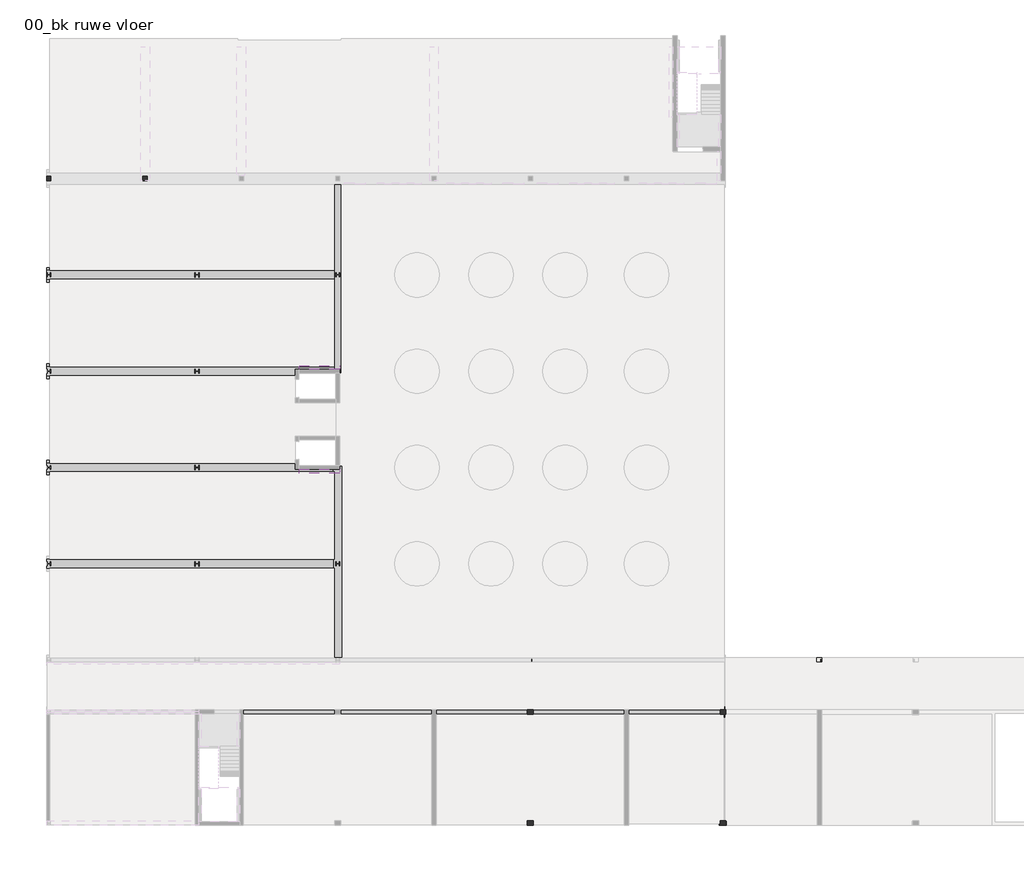
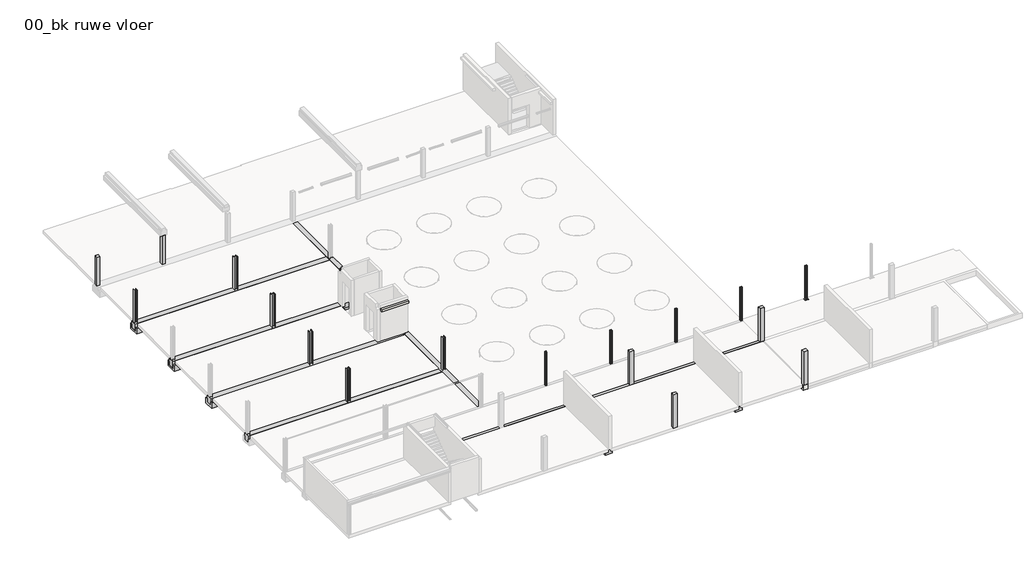
# One storey, part 5 of 6: 17 columns, 12 beams, 2 footings, 2 walls.
"""IFC4 building model written with IfcOpenShell, lengths in millimetres."""

import ifcopenshell
import ifcopenshell.guid

model = None  # the IFC model being written
_history = None  # IfcOwnerHistory: only IFC2X3 demands one
_inside = {}  # id of a spatial element -> (the spatial element, [elements in it])
_under = {}  # id of a project, library or spatial element -> (it, [spatial elements below it])
_declared = {}  # id of a project -> (the project, [libraries it declares])
_typed = {}  # id of a type object -> (the type object, [elements of that type])
_made_of = {}  # id of a material, layer set ... -> (it, [elements and type objects made of it])


def new_model(schema):
    """Start an empty IFC model of exactly this schema.

    Asked for "IFC4X3", IfcOpenShell would pick the latest addendum, in which some entities
    have other attributes; the version numbers below select the first issue.
    IFC2X3 requires an IfcOwnerHistory on every rooted entity: one is made here for all.
    """
    global model, _history
    if schema == "IFC4X3":
        model = ifcopenshell.file(schema_version=(4, 3, 0, 0))
    else:
        model = ifcopenshell.file(schema=schema)
    _inside.clear()
    _under.clear()
    _declared.clear()
    _typed.clear()
    _made_of.clear()
    _history = None
    if model.schema == "IFC2X3":
        org = make("IfcOrganization", Name="unknown")
        user = make(
            "IfcPersonAndOrganization",
            ThePerson=make("IfcPerson", FamilyName="unknown"),
            TheOrganization=org,
        )
        app = make(
            "IfcApplication",
            ApplicationDeveloper=org,
            Version="unknown",
            ApplicationFullName="unknown",
            ApplicationIdentifier="unknown",
        )
        _history = make(
            "IfcOwnerHistory",
            OwningUser=user,
            OwningApplication=app,
            ChangeAction="ADDED",
            CreationDate=0,
        )
    return model


def make(cls, **values):
    """One entity of the class cls with the attributes given. An attribute that is None is left unset."""
    return model.create_entity(
        cls, **{name: value for name, value in values.items() if value is not None}
    )


def rooted(cls, **values):
    """An entity with a GlobalId (a new one), such as an element, a storey or a relation."""
    return make(cls, GlobalId=ifcopenshell.guid.new(), OwnerHistory=_history, **values)


def si_unit(unit_type, name, prefix=None):
    """IfcSIUnit, for example si_unit("LENGTHUNIT", "METRE", prefix="MILLI")."""
    return make("IfcSIUnit", UnitType=unit_type, Prefix=prefix, Name=name)


def assignment(units):
    """IfcUnitAssignment: the units of a project."""
    return None if units is None else make("IfcUnitAssignment", Units=units)


def point(xyz):
    """IfcCartesianPoint."""
    return None if xyz is None else make("IfcCartesianPoint", Coordinates=xyz)


def direction(xyz):
    """IfcDirection."""
    return None if xyz is None else make("IfcDirection", DirectionRatios=xyz)


def frame(location, z_axis=None, x_axis=None):
    """IfcAxis2Placement3D, a coordinate frame: its origin and axes. An axis left out is left unset."""
    return make(
        "IfcAxis2Placement3D",
        Location=point(location),
        Axis=direction(z_axis),
        RefDirection=direction(x_axis),
    )


def frame_2d(location, x_axis=None):
    """IfcAxis2Placement2D, a coordinate frame in the plane: its origin and x axis."""
    return make(
        "IfcAxis2Placement2D", Location=point(location), RefDirection=direction(x_axis)
    )


def origin():
    """The frame at (0, 0, 0) with its axes left unset."""
    return frame((0.0, 0.0, 0.0))


def place(relative_to, where):
    """IfcLocalPlacement: puts the frame where relative to a parent placement (None: the world)."""
    return make(
        "IfcLocalPlacement", PlacementRelTo=relative_to, RelativePlacement=where
    )


def context(
    kind, dimensions, precision=None, world=None, true_north=None, identifier=None
):
    """IfcGeometricRepresentationContext, for example the 3D "Model" context."""
    return make(
        "IfcGeometricRepresentationContext",
        ContextIdentifier=identifier,
        ContextType=kind,
        CoordinateSpaceDimension=dimensions,
        Precision=precision,
        WorldCoordinateSystem=world,
        TrueNorth=true_north,
    )


def project(units=None, contexts=None):
    """IfcProject with its units and contexts."""
    return rooted(
        "IfcProject",
        Name="project",
        RepresentationContexts=contexts,
        UnitsInContext=assignment(units),
    )


def spatial(cls, under=None, at=None, **own):
    """A site, building, storey or space (cls), placed at a placement, below another one or the project."""
    s = rooted(cls, ObjectPlacement=at, **own)
    if under is not None:
        _under.setdefault(under.id(), (under, []))[1].append(s)
    return s


def polyline(points):
    """IfcPolyline through the points."""
    return make("IfcPolyline", Points=[point(p) for p in points])


def circle_curve(where, radius):
    """IfcCircle in the frame where."""
    return make("IfcCircle", Position=where, Radius=radius)


def trimmed(basis, trim1, trim2, sense, master):
    """IfcTrimmedCurve: the piece of a basis curve between two trims."""
    return make(
        "IfcTrimmedCurve",
        BasisCurve=basis,
        Trim1=trim1,
        Trim2=trim2,
        SenseAgreement=sense,
        MasterRepresentation=master,
    )


def segment(curve, same_sense, transition):
    """IfcCompositeCurveSegment."""
    return make(
        "IfcCompositeCurveSegment",
        Transition=transition,
        SameSense=same_sense,
        ParentCurve=curve,
    )


def composite_curve(segments, self_intersect=None):
    """IfcCompositeCurve: segments joined end to end."""
    return make("IfcCompositeCurve", Segments=segments, SelfIntersect=self_intersect)


def outline(outer, holes=None, kind="AREA"):
    """IfcArbitraryClosedProfileDef: a profile drawn as a closed curve; with holes, ...WithVoids."""
    if holes is None:
        return make("IfcArbitraryClosedProfileDef", ProfileType=kind, OuterCurve=outer)
    return make(
        "IfcArbitraryProfileDefWithVoids",
        ProfileType=kind,
        OuterCurve=outer,
        InnerCurves=holes,
    )


def extrude(swept, where, along, depth):
    """IfcExtrudedAreaSolid: the profile swept, set in the frame where, extruded along a direction by depth."""
    return make(
        "IfcExtrudedAreaSolid",
        SweptArea=swept,
        Position=where,
        ExtrudedDirection=direction(along),
        Depth=depth,
    )


def faces_of(points, faces, orient=None, outer=None):
    """IfcFace entities. A face is a list of loops; a loop is a list of indices into points, from 0.

    orient and outer hold one flag for each loop. By default every Orientation is true, the
    first loop of a face is its IfcFaceOuterBound and the others are IfcFaceBound.
    """
    made = []
    for i, loops in enumerate(faces):
        bounds = []
        for j, loop in enumerate(loops):
            is_outer = j == 0 if outer is None else outer[i][j]
            bounds.append(
                make(
                    "IfcFaceOuterBound" if is_outer else "IfcFaceBound",
                    Bound=make("IfcPolyLoop", Polygon=[points[k] for k in loop]),
                    Orientation=True if orient is None else orient[i][j],
                )
            )
        made.append(make("IfcFace", Bounds=bounds))
    return made


def faceted_brep(points, faces, orient=None, outer=None, voids=None):
    """IfcFacetedBrep: a solid bounded by flat faces; with voids (closed shells), ...WithVoids."""
    shared = [point(p) for p in points]
    hull = make("IfcClosedShell", CfsFaces=faces_of(shared, faces, orient, outer))
    if voids is None:
        return make("IfcFacetedBrep", Outer=hull)
    return make(
        "IfcFacetedBrepWithVoids",
        Outer=hull,
        Voids=[
            make(cls, CfsFaces=faces_of(shared, fs, o, b)) for cls, fs, o, b in voids
        ],
    )


def shape(context_of_items, identifier, shape_type, items):
    """IfcShapeRepresentation: the items that make up one representation, for example the "Body"."""
    return make(
        "IfcShapeRepresentation",
        ContextOfItems=context_of_items,
        RepresentationIdentifier=identifier,
        RepresentationType=shape_type,
        Items=items,
    )


def source(mapping_origin, context_of_items, identifier, shape_type, items):
    """IfcRepresentationMap: a shape defined once, which mapped items show again and again."""
    return make(
        "IfcRepresentationMap",
        MappingOrigin=mapping_origin,
        MappedRepresentation=shape(context_of_items, identifier, shape_type, items),
    )


def transform(
    local_origin,
    x_axis=None,
    y_axis=None,
    z_axis=None,
    scale=None,
    scale2=None,
    scale3=None,
    uniform=True,
):
    """IfcCartesianTransformationOperator3D, or its non-uniform kind. x_axis, y_axis, z_axis: its Axis1, 2, 3."""
    if uniform:
        return make(
            "IfcCartesianTransformationOperator3D",
            Axis1=direction(x_axis),
            Axis2=direction(y_axis),
            LocalOrigin=point(local_origin),
            Scale=scale,
            Axis3=direction(z_axis),
        )
    return make(
        "IfcCartesianTransformationOperator3DnonUniform",
        Axis1=direction(x_axis),
        Axis2=direction(y_axis),
        LocalOrigin=point(local_origin),
        Scale=scale,
        Axis3=direction(z_axis),
        Scale2=scale2,
        Scale3=scale3,
    )


def mapped(mapping_source, mapping_target):
    """IfcMappedItem: shows the shape of a source again, moved by a transform."""
    return make(
        "IfcMappedItem", MappingSource=mapping_source, MappingTarget=mapping_target
    )


def made_of(thing, what):
    """Note that an element or type object is made of a material, layer set ...; save() writes the relation."""
    if what is not None:
        _made_of.setdefault(what.id(), (what, []))[1].append(thing)
    return thing


def element(
    cls,
    number,
    at=None,
    inside=None,
    cuts=None,
    type_object=None,
    material=None,
    context=None,
    identifier="Body",
    shape_type=None,
    held_by="IfcProductDefinitionShape",
    body=None,
    shapes=None,
    **own,
):
    """One element of the class cls, such as IfcWall. Its Tag is "e" and its number.

    at: its placement. inside: the storey or other place that contains it. cuts: it is an
    opening in that element (IfcRelVoidsElement). A single representation is given by context,
    identifier, shape_type and body (its items); several are given by shapes. held_by: the class
    of the entity that holds the representations. save() writes the other relations.
    """
    e = rooted(cls, Tag="e%d" % number, ObjectPlacement=at, **own)
    if body is not None:
        shapes = [shape(context, identifier, shape_type, body)]
    if shapes is not None:
        e.Representation = make(held_by, Representations=shapes)
    if inside is not None:
        _inside.setdefault(inside.id(), (inside, []))[1].append(e)
    if cuts is not None:
        rooted(
            "IfcRelVoidsElement", RelatingBuildingElement=cuts, RelatedOpeningElement=e
        )
    if type_object is not None:
        _typed.setdefault(type_object.id(), (type_object, []))[1].append(e)
    return made_of(e, material)


def aggregate(whole, parts):
    """IfcRelAggregates: a whole, such as a stair, and the parts it consists of."""
    return rooted("IfcRelAggregates", RelatingObject=whole, RelatedObjects=parts)


def save(model, path):
    """Write the relations noted so far, then the file.

    IfcRelAggregates (storeys below a building ...), IfcRelContainedInSpatialStructure (elements
    in a storey), IfcRelDefinesByType, IfcRelAssociatesMaterial and IfcRelDeclares: one each for
    every whole, place, type object, material and project.
    """
    for whole, parts in _under.values():
        aggregate(whole, parts)
    for where, things in _inside.values():
        rooted(
            "IfcRelContainedInSpatialStructure",
            RelatedElements=things,
            RelatingStructure=where,
        )
    for kind, things in _typed.values():
        rooted("IfcRelDefinesByType", RelatedObjects=things, RelatingType=kind)
    for what, things in _made_of.values():
        rooted("IfcRelAssociatesMaterial", RelatedObjects=things, RelatingMaterial=what)
    for by, libraries in _declared.values():
        rooted("IfcRelDeclares", RelatingContext=by, RelatedDefinitions=libraries)
    model.write(path)


def column_d8346d76(model_context):
    return source(origin(), model_context, "Body", "SweptSolid", [
        extrude(outline(composite_curve([segment(trimmed(circle_curve(frame_2d((60.0, 60.0)), 20.0), [point((60.0, 80.0))], [point((80.0, 60.0))], False, "CARTESIAN"), True, "CONTINUOUS"), segment(polyline([(80.0, 60.0), (80.0, -60.0)]), True, "CONTINUOUS"), segment(trimmed(circle_curve(frame_2d((60.0, -60.0)), 20.0), [point((80.0, -60.0))], [point((60.0, -80.0))], False, "CARTESIAN"), True, "CONTINUOUS"), segment(polyline([(60.0, -80.0), (-60.0, -80.0)]), True, "CONTINUOUS"), segment(trimmed(circle_curve(frame_2d((-60.0, -60.0)), 20.0), [point((-60.0, -80.0))], [point((-80.0, -60.0))], False, "CARTESIAN"), True, "CONTINUOUS"), segment(polyline([(-80.0, -60.0), (-80.0, 60.0)]), True, "CONTINUOUS"), segment(trimmed(circle_curve(frame_2d((-60.0, 60.0)), 20.0), [point((-80.0, 60.0))], [point((-60.0, 80.0))], False, "CARTESIAN"), True, "CONTINUOUS"), segment(polyline([(-60.0, 80.0), (60.0, 80.0)]), True, "CONTINUOUS")], self_intersect=False), holes=[composite_curve([segment(polyline([(60.0, 72.0), (-60.0, 72.0)]), True, "CONTINUOUS"), segment(trimmed(circle_curve(frame_2d((-60.0, 60.0)), 12.0), [point((-60.0, 72.0))], [point((-72.0, 60.0))], True, "CARTESIAN"), True, "CONTINUOUS"), segment(polyline([(-72.0, 60.0), (-72.0, -60.0)]), True, "CONTINUOUS"), segment(trimmed(circle_curve(frame_2d((-60.0, -60.0)), 12.0), [point((-72.0, -60.0))], [point((-60.0, -72.0))], True, "CARTESIAN"), True, "CONTINUOUS"), segment(polyline([(-60.0, -72.0), (60.0, -72.0)]), True, "CONTINUOUS"), segment(trimmed(circle_curve(frame_2d((60.0, -60.0)), 12.0), [point((60.0, -72.0))], [point((72.0, -60.0))], True, "CARTESIAN"), True, "CONTINUOUS"), segment(polyline([(72.0, -60.0), (72.0, 60.0)]), True, "CONTINUOUS"), segment(trimmed(circle_curve(frame_2d((60.0, 60.0)), 12.0), [point((72.0, 60.0))], [point((60.0, 72.0))], True, "CARTESIAN"), True, "CONTINUOUS")], self_intersect=False)]), frame((0.0, 0.0, -40.0), z_axis=(0.0, 0.0, 1.0), x_axis=(1.0, 0.0, 0.0)), (0.0, 0.0, 1.0), 3510.0),
    ])


model = new_model("IFC4")

# Units and contexts
model_context = context("Model", 3, world=origin())
ifc_project = project(units=[si_unit("LENGTHUNIT", "METRE", prefix="MILLI")], contexts=[model_context])

# Site, building, storey
site = spatial("IfcSite", under=ifc_project)
building = spatial("IfcBuilding", under=site)
storey = spatial("IfcBuildingStorey", under=building, Name="00_bk ruwe vloer", Elevation=-70.0)

# Beams
placement = place(None, origin())
element("IfcBeam", 1, ObjectType="NLRS_28_SF_LIB_balk dubbele sponning beton prefab-CWV-MMBC-SRP_gen_rsf : balk beton prefab_gen__bxh 700x700 met inkassing bxh 200x320", at=placement, inside=storey, context=model_context, shape_type="Brep", body=[
    faceted_brep([(52150.0, 7650.0, -70.0), (52150.0, 7350.0, -70.0), (52150.0, 7350.0, -390.0), (52150.0, 7150.0, -390.0), (52150.0, 7150.0, -770.0), (52150.0, 7850.0, -770.0), (52150.0, 7850.0, -390.0), (52150.0, 7650.0, -390.0), (52090.0, 7650.0, -70.0), (51800.0, 7650.0, -70.0), (39200.0, 7650.0, -70.0), (38800.0, 7650.0, -70.0), (26200.0, 7650.0, -70.0), (25800.0, 7650.0, -70.0), (19625.0, 7650.0, -70.0), (19375.0, 7650.0, -70.0), (19375.0, 7400.0, -70.0), (19375.0, 7350.0, -70.0), (25800.0, 7350.0, -70.0), (26200.0, 7350.0, -70.0), (32350.0, 7350.0, -70.0), (32650.0, 7350.0, -70.0), (38800.0, 7350.0, -70.0), (39200.0, 7350.0, -70.0), (45350.0, 7350.0, -70.0), (45650.0, 7350.0, -70.0), (51800.0, 7350.0, -70.0), (52050.0, 7350.0, -70.0), (19375.0, 7350.0, -390.0), (19625.0, 7350.0, -390.0), (32350.0, 7350.0, -390.0), (32650.0, 7350.0, -390.0), (45350.0, 7350.0, -390.0), (45650.0, 7350.0, -390.0), (52050.0, 7350.0, -390.0), (19625.0, 7175.0, -390.0), (19625.0, 7150.0, -390.0), (32150.0, 7150.0, -390.0), (32175.0, 7150.0, -390.0), (32350.0, 7150.0, -390.0), (32650.0, 7150.0, -390.0), (32825.0, 7150.0, -390.0), (32850.0, 7150.0, -390.0), (45150.0, 7150.0, -390.0), (45175.0, 7150.0, -390.0), (45350.0, 7150.0, -390.0), (45650.0, 7150.0, -390.0), (45825.0, 7150.0, -390.0), (45850.0, 7150.0, -390.0), (51850.0, 7150.0, -390.0), (51875.0, 7150.0, -390.0), (52050.0, 7150.0, -390.0), (19625.0, 7150.0, -770.0), (32150.0, 7150.0, -770.0), (32850.0, 7150.0, -770.0), (45150.0, 7150.0, -770.0), (45850.0, 7150.0, -770.0), (51850.0, 7150.0, -770.0), (19625.0, 7650.0, -770.0), (19375.0, 7650.0, -770.0), (19375.0, 7850.0, -770.0), (51850.0, 7850.0, -770.0), (19375.0, 7850.0, -390.0), (51850.0, 7850.0, -390.0), (51875.0, 7850.0, -390.0), (52090.0, 7850.0, -390.0), (19375.0, 7825.0, -390.0), (19375.0, 7650.0, -390.0), (19625.0, 7650.0, -390.0), (52090.0, 7650.0, -390.0), (19625.0, 7650.0, -390.0)], [[[0, 1, 2, 3, 4, 5, 6, 7]], [[1, 0, 8, 9, 10, 11, 12, 13, 14, 15, 16, 17, 18, 19, 20, 21, 22, 23, 24, 25, 26, 27]], [[2, 1, 27, 26, 25, 24, 23, 22, 21, 20, 19, 18, 17, 28, 29, 30, 31, 32, 33, 34]], [[3, 2, 34, 33, 32, 31, 30, 29, 35, 36, 37, 38, 39, 40, 41, 42, 43, 44, 45, 46, 47, 48, 49, 50, 51]], [[4, 3, 51, 50, 49, 48, 47, 46, 45, 44, 43, 42, 41, 40, 39, 38, 37, 36, 52, 53, 54, 55, 56, 57]], [[5, 4, 57, 56, 55, 54, 53, 52, 58, 59, 60, 61]], [[6, 5, 61, 60, 62, 63, 64, 65]], [[7, 6, 65, 64, 63, 62, 66, 67, 68, 69]], [[0, 7, 69, 68, 67, 15, 14, 13, 12, 11, 10, 9, 8]], [[17, 16, 15, 67, 28]], [[29, 70, 58, 52, 36, 35]], [[67, 70, 29, 28]], [[70, 67, 59, 58]], [[62, 60, 59, 67, 66]]]),
])
element("IfcBeam", 2, ObjectType="NLRS_28_SF_LIB_balk dubbele sponning beton ihwg-CWV-MMBC-SRP_gen_rsf : balk beton ihwg_gen__bxh 1000x900 met inkassing bxh 200x320", at=placement, inside=storey, context=model_context, shape_type="Brep", body=[
    faceted_brep([(6350.0, 17200.0, -70.0), (6350.0, 17800.0, -70.0), (6350.0, 17800.0, -390.0), (6350.0, 17800.0, -770.0), (6350.0, 17200.0, -770.0), (6350.0, 17200.0, -390.0), (6550.0, 17200.0, -70.0), (25700.0, 17200.0, -70.0), (25700.0, 17800.0, -70.0), (6550.0, 17800.0, -70.0), (25500.0, 17200.0, -770.0), (25500.0, 17200.0, -390.0), (25550.0, 17200.0, -390.0), (25700.0, 17200.0, -390.0), (25700.0, 17800.0, -390.0), (25550.0, 17800.0, -390.0), (25500.0, 17800.0, -390.0), (25500.0, 17800.0, -770.0)], [[[0, 1, 2, 3, 4, 5]], [[1, 0, 6, 7, 8, 9]], [[0, 5, 4, 10, 11, 12, 13, 7, 6]], [[3, 2, 1, 9, 8, 14, 15, 16, 17]], [[4, 3, 17, 10]], [[16, 11, 10, 17]], [[14, 13, 12, 11, 16, 15]], [[13, 14, 8, 7]]]),
])
element("IfcBeam", 3, ObjectType="NLRS_28_SF_LIB_balk dubbele sponning beton ihwg-CWV-MMBC-SRP_gen_rsf : balk beton ihwg_gen__bxh 1000x900 met inkassing bxh 200x320", at=placement, inside=storey, context=model_context, shape_type="Brep", body=[
    faceted_brep([(6350.0, 23700.0, -70.0), (6350.0, 24300.0, -70.0), (6350.0, 24300.0, -390.0), (6350.0, 24300.0, -770.0), (6350.0, 23700.0, -770.0), (6350.0, 23700.0, -390.0), (6550.0, 23700.0, -70.0), (25700.0, 23700.0, -70.0), (25700.0, 23875.0, -70.0), (23375.0, 23875.0, -70.0), (23125.0, 23875.0, -70.0), (23125.0, 24300.0, -70.0), (6550.0, 24300.0, -70.0), (25500.0, 23700.0, -770.0), (25500.0, 23700.0, -390.0), (25550.0, 23700.0, -390.0), (25700.0, 23700.0, -390.0), (23125.0, 24300.0, -390.0), (23125.0, 24300.0, -770.0), (23125.0, 23875.0, -770.0), (23375.0, 23875.0, -770.0), (25500.0, 23875.0, -770.0), (25500.0, 23875.0, -390.0), (25700.0, 23875.0, -390.0)], [[[0, 1, 2, 3, 4, 5]], [[1, 0, 6, 7, 8, 9, 10, 11, 12]], [[0, 5, 4, 13, 14, 15, 16, 7, 6]], [[3, 2, 1, 12, 11, 17, 18]], [[4, 3, 18, 19, 20, 21, 13]], [[17, 11, 10, 19, 18]], [[22, 14, 13, 21]], [[14, 22, 23, 16, 15]], [[16, 23, 8, 7]], [[19, 10, 9, 8, 23, 22, 21, 20]]]),
])
element("IfcBeam", 4, ObjectType="NLRS_28_SF_LIB_balk dubbele sponning beton ihwg-CWV-MMBC-SRP_gen_rsf : balk beton ihwg_gen__bxh 1000x900 met inkassing bxh 200x320", at=placement, inside=storey, context=model_context, shape_type="Brep", body=[
    faceted_brep([(25750.0, 30800.0, -390.0), (25750.0, 30800.0, -70.0), (25750.0, 30625.0, -70.0), (25750.0, 30625.0, -390.0), (6350.0, 30200.0, -70.0), (6350.0, 30800.0, -70.0), (6350.0, 30800.0, -390.0), (6350.0, 30800.0, -770.0), (6350.0, 30200.0, -770.0), (6350.0, 30200.0, -390.0), (6550.0, 30200.0, -70.0), (23125.0, 30200.0, -70.0), (23375.0, 30200.0, -70.0), (23375.0, 30375.0, -70.0), (23375.0, 30625.0, -70.0), (6550.0, 30800.0, -70.0), (23375.0, 30200.0, -770.0), (23375.0, 30200.0, -390.0), (25550.0, 30800.0, -390.0), (25550.0, 30800.0, -770.0), (25550.0, 30625.0, -770.0), (23375.0, 30625.0, -770.0), (25550.0, 30625.0, -390.0)], [[[0, 1, 2, 3]], [[4, 5, 6, 7, 8, 9]], [[5, 4, 10, 11, 12, 13, 14, 2, 1, 15]], [[4, 9, 8, 16, 17, 12, 11, 10]], [[1, 0, 18, 19, 7, 6, 5, 15]], [[7, 19, 20, 21, 16, 8]], [[14, 21, 20, 22, 3, 2]], [[21, 14, 13, 12, 17, 16]], [[18, 22, 20, 19]], [[22, 18, 0, 3]]]),
])
element("IfcBeam", 5, ObjectType="NLRS_28_SF_LIB_balk dubbele sponning beton ihwg-CWV-MMBC-SRP_gen_rsf : balk beton ihwg_gen__bxh 1000x900 met inkassing bxh 200x320", at=placement, inside=storey, context=model_context, shape_type="Brep", body=[
    faceted_brep([(6350.0, 36700.0, -70.0), (6350.0, 37300.0, -70.0), (6350.0, 37300.0, -390.0), (6350.0, 37300.0, -770.0), (6350.0, 36700.0, -770.0), (6350.0, 36700.0, -390.0), (6550.0, 36700.0, -70.0), (25750.0, 36700.0, -70.0), (25750.0, 37300.0, -70.0), (6550.0, 37300.0, -70.0), (25550.0, 36700.0, -770.0), (25550.0, 36700.0, -390.0), (25750.0, 36700.0, -390.0), (25550.0, 37300.0, -770.0), (25750.0, 37300.0, -390.0), (25550.0, 37300.0, -390.0)], [[[0, 1, 2, 3, 4, 5]], [[1, 0, 6, 7, 8, 9]], [[4, 10, 11, 12, 7, 6, 0, 5]], [[13, 3, 2, 1, 9, 8, 14, 15]], [[3, 13, 10, 4]], [[15, 11, 10, 13]], [[11, 15, 14, 12]], [[12, 14, 8, 7]]]),
])
element("IfcBeam", 6, ObjectType="NLRS_28_SF_LIB_balkbodem beton prefab-CWV-MMBC-SRP_gen_rsf : balkbodem beton prefab_gen__bxhxdk 1000x580x200", at=placement, inside=storey, context=model_context, shape_type="Brep", body=[
    faceted_brep([(25550.0, 36500.0, -390.0), (25550.0, 36500.0, -970.0), (25550.0, 37500.0, -970.0), (25550.0, 37500.0, -390.0), (25550.0, 37300.0, -390.0), (25550.0, 37300.0, -770.0), (25550.0, 36700.0, -770.0), (25550.0, 36700.0, -390.0), (6350.0, 36500.0, -390.0), (6350.0, 36700.0, -390.0), (6350.0, 36700.0, -770.0), (6350.0, 37300.0, -770.0), (6350.0, 37300.0, -390.0), (6350.0, 37500.0, -390.0), (6350.0, 37500.0, -970.0), (6350.0, 36500.0, -970.0), (6650.0, 36500.0, -390.0), (6550.0, 36500.0, -390.0), (6650.0, 36500.0, -970.0), (6650.0, 37500.0, -970.0), (6550.0, 37500.0, -390.0), (6650.0, 37500.0, -390.0), (6550.0, 37300.0, -390.0), (6550.0, 36700.0, -390.0)], [[[0, 1, 2, 3, 4, 5, 6, 7]], [[8, 9, 10, 11, 12, 13, 14, 15]], [[1, 0, 16, 17, 8, 15, 18]], [[2, 1, 18, 15, 14, 19]], [[3, 2, 19, 14, 13, 20, 21]], [[4, 3, 21, 20, 13, 12, 22]], [[5, 4, 22, 12, 11]], [[6, 5, 11, 10]], [[7, 6, 10, 9, 23]], [[0, 7, 23, 9, 8, 17, 16]]]),
])
element("IfcBeam", 7, ObjectType="NLRS_28_SF_LIB_balkbodem beton prefab-CWV-MMBC-SRP_gen_rsf : balkbodem beton prefab_gen__bxhxdk 1000x580x200", at=placement, inside=storey, context=model_context, shape_type="Brep", body=[
    faceted_brep([(25550.0, 31000.0, -970.0), (25550.0, 31000.0, -390.0), (25550.0, 30800.0, -390.0), (25550.0, 30800.0, -770.0), (25550.0, 30625.0, -770.0), (25550.0, 30625.0, -970.0), (6350.0, 30000.0, -390.0), (6350.0, 30200.0, -390.0), (6350.0, 30200.0, -770.0), (6350.0, 30800.0, -770.0), (6350.0, 30800.0, -390.0), (6350.0, 31000.0, -390.0), (6350.0, 31000.0, -970.0), (6350.0, 30000.0, -970.0), (6650.0, 30000.0, -970.0), (23125.0, 30000.0, -970.0), (23375.0, 30000.0, -970.0), (23375.0, 30000.0, -390.0), (23125.0, 30000.0, -390.0), (6650.0, 30000.0, -390.0), (6550.0, 30000.0, -390.0), (6650.0, 31000.0, -970.0), (23375.0, 30625.0, -970.0), (6550.0, 31000.0, -390.0), (6650.0, 31000.0, -390.0), (6550.0, 30800.0, -390.0), (23375.0, 30200.0, -770.0), (23375.0, 30625.0, -770.0), (6550.0, 30200.0, -390.0), (23125.0, 30200.0, -390.0), (23375.0, 30200.0, -390.0)], [[[0, 1, 2, 3, 4, 5]], [[6, 7, 8, 9, 10, 11, 12, 13]], [[6, 13, 14, 15, 16, 17, 18, 19, 20]], [[13, 12, 21, 0, 5, 22, 16, 15, 14]], [[1, 0, 21, 12, 11, 23, 24]], [[2, 1, 24, 23, 11, 10, 25]], [[3, 2, 25, 10, 9]], [[9, 8, 26, 27, 4, 3]], [[8, 7, 28, 29, 30, 26]], [[7, 6, 20, 19, 18, 17, 30, 29, 28]], [[27, 22, 5, 4]], [[17, 16, 22, 27, 26, 30]]]),
])
element("IfcBeam", 8, ObjectType="NLRS_28_SF_LIB_balkbodem beton prefab-CWV-MMBC-SRP_gen_rsf : balkbodem beton prefab_gen__bxhxdk 1000x580x200", at=placement, inside=storey, context=model_context, shape_type="Brep", body=[
    faceted_brep([(25550.0, 23500.0, -390.0), (25550.0, 23500.0, -970.0), (25550.0, 23875.0, -970.0), (25550.0, 23875.0, -770.0), (25550.0, 23700.0, -770.0), (25550.0, 23700.0, -390.0), (6350.0, 23500.0, -390.0), (6350.0, 23700.0, -390.0), (6350.0, 23700.0, -770.0), (6350.0, 24300.0, -770.0), (6350.0, 24300.0, -390.0), (6350.0, 24500.0, -390.0), (6350.0, 24500.0, -970.0), (6350.0, 23500.0, -970.0), (25500.0, 23500.0, -390.0), (6650.0, 23500.0, -390.0), (6550.0, 23500.0, -390.0), (6650.0, 23500.0, -970.0), (25500.0, 23500.0, -970.0), (6650.0, 24500.0, -970.0), (23125.0, 24500.0, -970.0), (23375.0, 24500.0, -970.0), (23375.0, 23875.0, -970.0), (6550.0, 24500.0, -390.0), (6650.0, 24500.0, -390.0), (23125.0, 24500.0, -390.0), (23375.0, 24500.0, -390.0), (6550.0, 24300.0, -390.0), (23125.0, 24300.0, -390.0), (23375.0, 24300.0, -390.0), (23125.0, 24300.0, -770.0), (23375.0, 24300.0, -770.0), (25500.0, 23700.0, -770.0), (25500.0, 23875.0, -770.0), (23375.0, 23875.0, -770.0), (6550.0, 23700.0, -390.0), (25500.0, 23700.0, -390.0)], [[[0, 1, 2, 3, 4, 5]], [[6, 7, 8, 9, 10, 11, 12, 13]], [[1, 0, 14, 15, 16, 6, 13, 17, 18]], [[13, 12, 19, 20, 21, 22, 2, 1, 18, 17]], [[12, 11, 23, 24, 25, 26, 21, 20, 19]], [[11, 10, 27, 28, 29, 26, 25, 24, 23]], [[10, 9, 30, 31, 29, 28, 27]], [[9, 8, 32, 4, 3, 33, 34, 31, 30]], [[5, 4, 32, 8, 7, 35, 36]], [[0, 5, 36, 35, 7, 6, 16, 15, 14]], [[22, 34, 33, 3, 2]], [[21, 26, 29, 31, 34, 22]]]),
])
element("IfcBeam", 9, ObjectType="NLRS_28_SF_LIB_balk dubbele sponning beton ihwg-CWV-MMBC-SRP_gen_rsf : balk beton ihwg_gen__bxh 900x900 met inkassing bxh 200x320", at=placement, inside=storey, context=model_context, shape_type="Brep", body=[
    faceted_brep([(25750.0, 43100.0, -70.0), (26250.0, 43100.0, -70.0), (26250.0, 43100.0, -390.0), (25750.0, 43100.0, -390.0), (25750.0, 30375.0, -70.0), (25750.0, 30375.0, -390.0), (25550.0, 30375.0, -390.0), (25550.0, 30375.0, -970.0), (25875.0, 30375.0, -970.0), (25875.0, 30375.0, -390.0), (26125.0, 30375.0, -390.0), (26125.0, 30375.0, -970.0), (26450.0, 30375.0, -970.0), (26450.0, 30375.0, -390.0), (26425.0, 30375.0, -390.0), (26250.0, 30375.0, -390.0), (26250.0, 30375.0, -70.0), (25750.0, 37300.0, -70.0), (25750.0, 36700.0, -70.0), (25750.0, 30800.0, -70.0), (25750.0, 30625.0, -70.0), (26250.0, 42900.0, -390.0), (26450.0, 42900.0, -390.0), (26425.0, 42900.0, -390.0), (26450.0, 42900.0, -970.0), (26125.0, 30625.0, -970.0), (25875.0, 30625.0, -970.0), (25550.0, 30625.0, -970.0), (25550.0, 36500.0, -970.0), (25550.0, 37500.0, -970.0), (25550.0, 42900.0, -970.0), (25550.0, 30625.0, -390.0), (25550.0, 30800.0, -390.0), (25550.0, 36500.0, -390.0), (25550.0, 36700.0, -390.0), (25550.0, 37300.0, -390.0), (25550.0, 37500.0, -390.0), (25550.0, 42900.0, -390.0), (25750.0, 30625.0, -390.0), (25750.0, 30800.0, -390.0), (25750.0, 36700.0, -390.0), (25750.0, 37300.0, -390.0), (25750.0, 42900.0, -390.0), (26125.0, 30625.0, -390.0), (25875.0, 30625.0, -390.0)], [[[0, 1, 2, 3]], [[4, 5, 6, 7, 8, 9, 10, 11, 12, 13, 14, 15, 16]], [[1, 0, 17, 18, 19, 20, 4, 16]], [[2, 1, 16, 15, 21]], [[21, 15, 14, 13, 22, 23]], [[13, 12, 24, 22]], [[12, 11, 25, 26, 8, 7, 27, 28, 29, 30, 24]], [[7, 6, 31, 32, 33, 34, 35, 36, 37, 30, 29, 28, 27]], [[6, 5, 38, 39, 40, 41, 42, 37, 36, 35, 34, 33, 32, 31]], [[0, 3, 42, 41, 40, 39, 38, 5, 4, 20, 19, 18, 17]], [[3, 2, 21, 42]], [[22, 24, 30, 37, 42, 21, 23]], [[10, 43, 25, 11]], [[26, 44, 9, 8]], [[43, 44, 26, 25]], [[44, 43, 10, 9]]]),
])
element("IfcBeam", 10, ObjectType="NLRS_28_SF_LIB_balk dubbele sponning beton ihwg-CWV-MMBC-SRP_gen_rsf : balk beton ihwg_gen__bxh 1000x900 met inkassing bxh 200x320", at=placement, inside=storey, context=model_context, shape_type="Brep", body=[
    faceted_brep([(26300.0, 24125.0, -70.0), (26300.0, 24125.0, -390.0), (26425.0, 24125.0, -390.0), (26500.0, 24125.0, -390.0), (26500.0, 24125.0, -970.0), (26125.0, 24125.0, -970.0), (26125.0, 24125.0, -390.0), (25875.0, 24125.0, -390.0), (25875.0, 24125.0, -70.0), (26300.0, 11150.0, -390.0), (26300.0, 11150.0, -70.0), (25750.0, 11150.0, -70.0), (25750.0, 11150.0, -390.0), (25875.0, 23875.0, -70.0), (25700.0, 23875.0, -70.0), (25700.0, 23700.0, -70.0), (25750.0, 23700.0, -70.0), (25750.0, 17800.0, -70.0), (25700.0, 17800.0, -70.0), (25700.0, 17200.0, -70.0), (25750.0, 17200.0, -70.0), (26300.0, 11350.0, -390.0), (26425.0, 11350.0, -390.0), (26500.0, 11350.0, -390.0), (26500.0, 11350.0, -970.0), (26125.0, 23875.0, -970.0), (25500.0, 11350.0, -970.0), (25500.0, 17000.0, -970.0), (25550.0, 17000.0, -970.0), (25550.0, 18000.0, -970.0), (25500.0, 18000.0, -970.0), (25500.0, 23500.0, -970.0), (25550.0, 23500.0, -970.0), (25550.0, 23875.0, -970.0), (25500.0, 23875.0, -390.0), (25500.0, 23875.0, -770.0), (25500.0, 23700.0, -770.0), (25500.0, 23700.0, -390.0), (25750.0, 11350.0, -390.0), (25750.0, 17200.0, -390.0), (25700.0, 17200.0, -390.0), (25700.0, 17800.0, -390.0), (25750.0, 17800.0, -390.0), (25750.0, 23700.0, -390.0), (25700.0, 23700.0, -390.0), (25700.0, 23875.0, -390.0), (25550.0, 23700.0, -390.0), (25550.0, 23500.0, -390.0), (25500.0, 23500.0, -390.0), (25500.0, 18000.0, -390.0), (25550.0, 18000.0, -390.0), (25550.0, 17800.0, -390.0), (25500.0, 17800.0, -390.0), (25500.0, 17200.0, -390.0), (25550.0, 17200.0, -390.0), (25550.0, 17000.0, -390.0), (25500.0, 17000.0, -390.0), (25500.0, 11350.0, -390.0), (25550.0, 23700.0, -770.0), (25550.0, 23875.0, -770.0), (25550.0, 17200.0, -770.0), (25550.0, 17800.0, -770.0), (25500.0, 17800.0, -770.0), (25500.0, 17200.0, -770.0), (25875.0, 23875.0, -390.0), (26125.0, 23875.0, -390.0)], [[[0, 1, 2, 3, 4, 5, 6, 7, 8]], [[9, 10, 11, 12]], [[10, 0, 8, 13, 14, 15, 16, 17, 18, 19, 20, 11]], [[1, 0, 10, 9, 21]], [[1, 21, 22, 23, 3, 2]], [[4, 3, 23, 24]], [[25, 5, 4, 24, 26, 27, 28, 29, 30, 31, 32, 33]], [[34, 35, 36, 37]], [[38, 39, 40, 41, 42, 43, 44, 45, 34, 37, 46, 47, 48, 49, 50, 51, 52, 53, 54, 55, 56, 57]], [[44, 15, 14, 45]], [[24, 23, 22, 21, 38, 57, 26]], [[12, 38, 21, 9]], [[32, 47, 46, 58, 59, 33]], [[47, 32, 31, 48]], [[58, 46, 37, 36]], [[28, 55, 54, 60, 61, 51, 50, 29]], [[55, 28, 27, 56]], [[29, 50, 49, 30]], [[51, 61, 62, 52]], [[60, 54, 53, 63]], [[20, 39, 38, 12, 11]], [[39, 20, 19, 40]], [[43, 42, 17, 16]], [[17, 42, 41, 18]], [[43, 16, 15, 44]], [[45, 14, 13, 64, 65, 25, 33, 59, 35, 34]], [[25, 65, 6, 5]], [[65, 64, 7, 6]], [[58, 36, 35, 59]], [[61, 60, 63, 62]], [[48, 31, 30, 49]], [[53, 52, 62, 63]], [[26, 57, 56, 27]], [[40, 19, 18, 41]], [[13, 8, 7, 64]]]),
])
element("IfcBeam", 11, ObjectType="NLRS_28_SF_LIB_balk dubbele sponning beton prefab-CWV-MMBC-SRP_gen_rsf : balk beton prefab_gen__bxh 700x700 met inkassing bxh 200x320", at=placement, inside=storey, context=model_context, shape_type="Brep", body=[
    faceted_brep([(32650.0, 7350.0, -70.0), (32350.0, 7350.0, -70.0), (32350.0, 150.0, -70.0), (32650.0, 150.0, -70.0), (32350.0, 7350.0, -390.0), (32350.0, 7150.0, -390.0), (32350.0, 150.0, -390.0), (32850.0, 7150.0, -390.0), (32825.0, 7150.0, -390.0), (32650.0, 7150.0, -390.0), (32650.0, 150.0, -390.0), (32850.0, 150.0, -390.0), (32150.0, 7150.0, -390.0), (32150.0, 7150.0, -770.0), (32150.0, 150.0, -770.0), (32150.0, 150.0, -390.0), (32850.0, 7150.0, -770.0), (32850.0, 150.0, -770.0), (32650.0, 7350.0, -390.0), (32175.0, 7150.0, -390.0)], [[[0, 1, 2, 3]], [[1, 4, 5, 6, 2]], [[7, 8, 9, 10, 11]], [[12, 13, 14, 15]], [[13, 16, 17, 14]], [[16, 7, 11, 17]], [[18, 0, 3, 10, 9]], [[1, 0, 18, 4]], [[5, 4, 18, 9]], [[13, 12, 19, 5, 9, 8, 7, 16]], [[19, 12, 15, 6, 5]], [[3, 2, 6, 15, 14, 17, 11, 10]]]),
])
element("IfcBeam", 12, ObjectType="NLRS_28_SF_LIB_balk dubbele sponning beton prefab-CWV-MMBC-SRP_gen_rsf : balk beton prefab_gen__bxh 700x700 met inkassing bxh 200x320", at=placement, inside=storey, context=model_context, shape_type="Brep", body=[
    faceted_brep([(45650.0, 7350.0, -70.0), (45350.0, 7350.0, -70.0), (45350.0, 150.0, -70.0), (45650.0, 150.0, -70.0), (45350.0, 7350.0, -390.0), (45350.0, 7150.0, -390.0), (45350.0, 150.0, -390.0), (45850.0, 7150.0, -390.0), (45825.0, 7150.0, -390.0), (45650.0, 7150.0, -390.0), (45650.0, 150.0, -390.0), (45850.0, 150.0, -390.0), (45150.0, 7150.0, -390.0), (45150.0, 7150.0, -770.0), (45150.0, 150.0, -770.0), (45150.0, 150.0, -390.0), (45850.0, 7150.0, -770.0), (45850.0, 150.0, -770.0), (45650.0, 7350.0, -390.0), (45175.0, 7150.0, -390.0)], [[[0, 1, 2, 3]], [[1, 4, 5, 6, 2]], [[7, 8, 9, 10, 11]], [[12, 13, 14, 15]], [[13, 16, 17, 14]], [[16, 7, 11, 17]], [[18, 0, 3, 10, 9]], [[1, 0, 18, 4]], [[5, 4, 18, 9]], [[13, 12, 19, 5, 9, 8, 7, 16]], [[19, 12, 15, 6, 5]], [[3, 2, 6, 15, 14, 17, 11, 10]]]),
])

# Columns
element("IfcColumn", 13, ObjectType="NLRS_28_SCO_TLB_stalen kolom HEA-BCPG-MMBS-SRP_gen_rsf : stalen kolom_gen__HEA 260", at=placement, inside=storey, context=model_context, shape_type="SweptSolid", body=[
    extrude(outline(composite_curve([segment(polyline([(6375.0, 37130.0), (6387.5, 37130.0), (6387.5, 37027.75)]), True, "CONTINUOUS"), segment(trimmed(circle_curve(frame_2d((6411.5, 37027.75)), 24.0), [point((6387.5, 37027.75))], [point((6411.5, 37003.75))], True, "CARTESIAN"), True, "CONTINUOUS"), segment(polyline([(6411.5, 37003.75), (6588.5, 37003.75)]), True, "CONTINUOUS"), segment(trimmed(circle_curve(frame_2d((6588.5, 37027.75)), 24.0), [point((6588.5, 37003.75))], [point((6612.5, 37027.75))], True, "CARTESIAN"), True, "CONTINUOUS"), segment(polyline([(6612.5, 37027.75), (6612.5, 37130.0), (6625.0, 37130.0), (6625.0, 36870.0), (6612.5, 36870.0), (6612.5, 36972.25)]), True, "CONTINUOUS"), segment(trimmed(circle_curve(frame_2d((6588.5, 36972.25)), 24.0), [point((6612.5, 36972.25))], [point((6588.5, 36996.25))], True, "CARTESIAN"), True, "CONTINUOUS"), segment(polyline([(6588.5, 36996.25), (6411.5, 36996.25)]), True, "CONTINUOUS"), segment(trimmed(circle_curve(frame_2d((6411.5, 36972.25)), 24.0), [point((6411.5, 36996.25))], [point((6387.5, 36972.25))], True, "CARTESIAN"), True, "CONTINUOUS"), segment(polyline([(6387.5, 36972.25), (6387.5, 36870.0), (6375.0, 36870.0), (6375.0, 37130.0)]), True, "CONTINUOUS")], self_intersect=False)), frame((0.0, 0.0, -40.0), z_axis=(0.0, 0.0, 1.0), x_axis=(1.0, 0.0, 0.0)), (0.0, 0.0, 1.0), 3420.0),
])
element("IfcColumn", 14, ObjectType="NLRS_28_SCO_TLB_vierkante kolom beton prefab-BCPG-MMBPC-SRP_gen_rsf : kolom vierkant beton prefab_gen__bxh 300x300", at=placement, inside=storey, context=model_context, shape_type="SweptSolid", body=[
    extrude(outline(polyline([(6350.0, 43650.0), (6650.0, 43650.0), (6650.0, 43350.0), (6350.0, 43350.0), (6350.0, 43650.0)])), frame((0.0, 0.0, -40.0), z_axis=(0.0, 0.0, 1.0), x_axis=(1.0, 0.0, 0.0)), (0.0, 0.0, 1.0), 3020.0),
])
element("IfcColumn", 15, ObjectType="NLRS_28_SCO_TLB_vierkante kolom beton prefab-BCPG-MMBPC-SRP_gen_rsf : kolom vierkant beton prefab_gen__bxh 300x300", at=placement, inside=storey, context=model_context, shape_type="SweptSolid", body=[
    extrude(outline(polyline([(13150.0, 43650.0), (13150.0, 43350.0), (12850.0, 43350.0), (12850.0, 43650.0), (13150.0, 43650.0)])), frame((0.0, 0.0, -40.0), z_axis=(0.0, 0.0, 1.0), x_axis=(1.0, 0.0, 0.0)), (0.0, 0.0, 1.0), 3020.0),
])
element("IfcColumn", 16, ObjectType="NLRS_28_SCO_TLB_stalen kolom HEB-BCPG-MMBS-SRP_gen_rsf : stalen kolom_gen__HEB 300", at=placement, inside=storey, context=model_context, shape_type="SweptSolid", body=[
    extrude(outline(composite_curve([segment(polyline([(16350.0, 17650.0), (16369.0, 17650.0), (16369.0, 17532.5)]), True, "CONTINUOUS"), segment(trimmed(circle_curve(frame_2d((16396.0, 17532.5)), 27.0), [point((16369.0, 17532.5))], [point((16396.0, 17505.5))], True, "CARTESIAN"), True, "CONTINUOUS"), segment(polyline([(16396.0, 17505.5), (16604.0, 17505.5)]), True, "CONTINUOUS"), segment(trimmed(circle_curve(frame_2d((16604.0, 17532.5)), 27.0), [point((16604.0, 17505.5))], [point((16631.0, 17532.5))], True, "CARTESIAN"), True, "CONTINUOUS"), segment(polyline([(16631.0, 17532.5), (16631.0, 17650.0), (16650.0, 17650.0), (16650.0, 17350.0), (16631.0, 17350.0), (16631.0, 17467.5)]), True, "CONTINUOUS"), segment(trimmed(circle_curve(frame_2d((16604.0, 17467.5)), 27.0), [point((16631.0, 17467.5))], [point((16604.0, 17494.5))], True, "CARTESIAN"), True, "CONTINUOUS"), segment(polyline([(16604.0, 17494.5), (16396.0, 17494.5)]), True, "CONTINUOUS"), segment(trimmed(circle_curve(frame_2d((16396.0, 17467.5)), 27.0), [point((16396.0, 17494.5))], [point((16369.0, 17467.5))], True, "CARTESIAN"), True, "CONTINUOUS"), segment(polyline([(16369.0, 17467.5), (16369.0, 17350.0), (16350.0, 17350.0), (16350.0, 17650.0)]), True, "CONTINUOUS")], self_intersect=False)), frame((0.0, 0.0, -40.0), z_axis=(0.0, 0.0, 1.0), x_axis=(1.0, 0.0, 0.0)), (0.0, 0.0, 1.0), 3420.0),
])
element("IfcColumn", 17, ObjectType="NLRS_28_SCO_TLB_stalen kolom HEB-BCPG-MMBS-SRP_gen_rsf : stalen kolom_gen__HEB 300", at=placement, inside=storey, context=model_context, shape_type="SweptSolid", body=[
    extrude(outline(composite_curve([segment(polyline([(16350.0, 24150.0), (16369.0, 24150.0), (16369.0, 24032.5)]), True, "CONTINUOUS"), segment(trimmed(circle_curve(frame_2d((16396.0, 24032.5)), 27.0), [point((16369.0, 24032.5))], [point((16396.0, 24005.5))], True, "CARTESIAN"), True, "CONTINUOUS"), segment(polyline([(16396.0, 24005.5), (16604.0, 24005.5)]), True, "CONTINUOUS"), segment(trimmed(circle_curve(frame_2d((16604.0, 24032.5)), 27.0), [point((16604.0, 24005.5))], [point((16631.0, 24032.5))], True, "CARTESIAN"), True, "CONTINUOUS"), segment(polyline([(16631.0, 24032.5), (16631.0, 24150.0), (16650.0, 24150.0), (16650.0, 23850.0), (16631.0, 23850.0), (16631.0, 23967.5)]), True, "CONTINUOUS"), segment(trimmed(circle_curve(frame_2d((16604.0, 23967.5)), 27.0), [point((16631.0, 23967.5))], [point((16604.0, 23994.5))], True, "CARTESIAN"), True, "CONTINUOUS"), segment(polyline([(16604.0, 23994.5), (16396.0, 23994.5)]), True, "CONTINUOUS"), segment(trimmed(circle_curve(frame_2d((16396.0, 23967.5)), 27.0), [point((16396.0, 23994.5))], [point((16369.0, 23967.5))], True, "CARTESIAN"), True, "CONTINUOUS"), segment(polyline([(16369.0, 23967.5), (16369.0, 23850.0), (16350.0, 23850.0), (16350.0, 24150.0)]), True, "CONTINUOUS")], self_intersect=False)), frame((0.0, 0.0, -40.0), z_axis=(0.0, 0.0, 1.0), x_axis=(1.0, 0.0, 0.0)), (0.0, 0.0, 1.0), 3420.0),
])
element("IfcColumn", 18, ObjectType="NLRS_28_SCO_TLB_stalen kolom HEB-BCPG-MMBS-SRP_gen_rsf : stalen kolom_gen__HEB 300", at=placement, inside=storey, context=model_context, shape_type="SweptSolid", body=[
    extrude(outline(composite_curve([segment(polyline([(16350.0, 30650.0), (16369.0, 30650.0), (16369.0, 30532.5)]), True, "CONTINUOUS"), segment(trimmed(circle_curve(frame_2d((16396.0, 30532.5)), 27.0), [point((16369.0, 30532.5))], [point((16396.0, 30505.5))], True, "CARTESIAN"), True, "CONTINUOUS"), segment(polyline([(16396.0, 30505.5), (16604.0, 30505.5)]), True, "CONTINUOUS"), segment(trimmed(circle_curve(frame_2d((16604.0, 30532.5)), 27.0), [point((16604.0, 30505.5))], [point((16631.0, 30532.5))], True, "CARTESIAN"), True, "CONTINUOUS"), segment(polyline([(16631.0, 30532.5), (16631.0, 30650.0), (16650.0, 30650.0), (16650.0, 30350.0), (16631.0, 30350.0), (16631.0, 30467.5)]), True, "CONTINUOUS"), segment(trimmed(circle_curve(frame_2d((16604.0, 30467.5)), 27.0), [point((16631.0, 30467.5))], [point((16604.0, 30494.5))], True, "CARTESIAN"), True, "CONTINUOUS"), segment(polyline([(16604.0, 30494.5), (16396.0, 30494.5)]), True, "CONTINUOUS"), segment(trimmed(circle_curve(frame_2d((16396.0, 30467.5)), 27.0), [point((16396.0, 30494.5))], [point((16369.0, 30467.5))], True, "CARTESIAN"), True, "CONTINUOUS"), segment(polyline([(16369.0, 30467.5), (16369.0, 30350.0), (16350.0, 30350.0), (16350.0, 30650.0)]), True, "CONTINUOUS")], self_intersect=False)), frame((0.0, 0.0, -40.0), z_axis=(0.0, 0.0, 1.0), x_axis=(1.0, 0.0, 0.0)), (0.0, 0.0, 1.0), 3420.0),
])
element("IfcColumn", 19, ObjectType="NLRS_28_SCO_TLB_stalen kolom HEB-BCPG-MMBS-SRP_gen_rsf : stalen kolom_gen__HEB 300", at=placement, inside=storey, context=model_context, shape_type="SweptSolid", body=[
    extrude(outline(composite_curve([segment(polyline([(16350.0, 37150.0), (16369.0, 37150.0), (16369.0, 37032.5)]), True, "CONTINUOUS"), segment(trimmed(circle_curve(frame_2d((16396.0, 37032.5)), 27.0), [point((16369.0, 37032.5))], [point((16396.0, 37005.5))], True, "CARTESIAN"), True, "CONTINUOUS"), segment(polyline([(16396.0, 37005.5), (16604.0, 37005.5)]), True, "CONTINUOUS"), segment(trimmed(circle_curve(frame_2d((16604.0, 37032.5)), 27.0), [point((16604.0, 37005.5))], [point((16631.0, 37032.5))], True, "CARTESIAN"), True, "CONTINUOUS"), segment(polyline([(16631.0, 37032.5), (16631.0, 37150.0), (16650.0, 37150.0), (16650.0, 36850.0), (16631.0, 36850.0), (16631.0, 36967.5)]), True, "CONTINUOUS"), segment(trimmed(circle_curve(frame_2d((16604.0, 36967.5)), 27.0), [point((16631.0, 36967.5))], [point((16604.0, 36994.5))], True, "CARTESIAN"), True, "CONTINUOUS"), segment(polyline([(16604.0, 36994.5), (16396.0, 36994.5)]), True, "CONTINUOUS"), segment(trimmed(circle_curve(frame_2d((16396.0, 36967.5)), 27.0), [point((16396.0, 36994.5))], [point((16369.0, 36967.5))], True, "CARTESIAN"), True, "CONTINUOUS"), segment(polyline([(16369.0, 36967.5), (16369.0, 36850.0), (16350.0, 36850.0), (16350.0, 37150.0)]), True, "CONTINUOUS")], self_intersect=False)), frame((0.0, 0.0, -40.0), z_axis=(0.0, 0.0, 1.0), x_axis=(1.0, 0.0, 0.0)), (0.0, 0.0, 1.0), 3420.0),
])
element("IfcColumn", 20, ObjectType="NLRS_28_SCO_TLB_stalen kolom HEA-BCPG-MMBS-SRP_gen_rsf : stalen kolom_gen__HEA 260", at=placement, inside=storey, context=model_context, shape_type="SweptSolid", body=[
    extrude(outline(composite_curve([segment(polyline([(25875.0, 17630.0), (25887.5, 17630.0), (25887.5, 17527.75)]), True, "CONTINUOUS"), segment(trimmed(circle_curve(frame_2d((25911.5, 17527.75)), 24.0), [point((25887.5, 17527.75))], [point((25911.5, 17503.75))], True, "CARTESIAN"), True, "CONTINUOUS"), segment(polyline([(25911.5, 17503.75), (26088.5, 17503.75)]), True, "CONTINUOUS"), segment(trimmed(circle_curve(frame_2d((26088.5, 17527.75)), 24.0), [point((26088.5, 17503.75))], [point((26112.5, 17527.75))], True, "CARTESIAN"), True, "CONTINUOUS"), segment(polyline([(26112.5, 17527.75), (26112.5, 17630.0), (26125.0, 17630.0), (26125.0, 17370.0), (26112.5, 17370.0), (26112.5, 17472.25)]), True, "CONTINUOUS"), segment(trimmed(circle_curve(frame_2d((26088.5, 17472.25)), 24.0), [point((26112.5, 17472.25))], [point((26088.5, 17496.25))], True, "CARTESIAN"), True, "CONTINUOUS"), segment(polyline([(26088.5, 17496.25), (25911.5, 17496.25)]), True, "CONTINUOUS"), segment(trimmed(circle_curve(frame_2d((25911.5, 17472.25)), 24.0), [point((25911.5, 17496.25))], [point((25887.5, 17472.25))], True, "CARTESIAN"), True, "CONTINUOUS"), segment(polyline([(25887.5, 17472.25), (25887.5, 17370.0), (25875.0, 17370.0), (25875.0, 17630.0)]), True, "CONTINUOUS")], self_intersect=False)), frame((0.0, 0.0, -40.0), z_axis=(0.0, 0.0, 1.0), x_axis=(1.0, 0.0, 0.0)), (0.0, 0.0, 1.0), 3420.0),
])
element("IfcColumn", 21, ObjectType="NLRS_28_SCO_TLB_vierkante kolom beton ihwg-BCPG-MMBC-SRP_gen_rsf : vierkante kolom beton ihwg_gen__bxh 400x300", at=placement, inside=storey, context=model_context, shape_type="SweptSolid", body=[
    extrude(outline(polyline([(39200.0, 150.0), (39200.0, -150.0), (38800.0, -150.0), (38800.0, 150.0), (39200.0, 150.0)])), frame((0.0, 0.0, -70.0), z_axis=(0.0, 0.0, 1.0), x_axis=(1.0, 0.0, 0.0)), (0.0, 0.0, 1.0), 3540.0),
])
element("IfcColumn", 22, ObjectType="NLRS_28_SCO_TLB_vierkante kolom beton ihwg-BCPG-MMBC-SRP_gen_rsf : vierkante kolom beton ihwg_gen__bxh 400x300", at=placement, inside=storey, context=model_context, shape_type="SweptSolid", body=[
    extrude(outline(polyline([(39200.0, 7650.0), (39200.0, 7350.0), (38800.0, 7350.0), (38800.0, 7650.0), (39200.0, 7650.0)])), frame((0.0, 0.0, -70.0), z_axis=(0.0, 0.0, 1.0), x_axis=(1.0, 0.0, 0.0)), (0.0, 0.0, 1.0), 3540.0),
])
element("IfcColumn", 23, ObjectType="NLRS_28_SCO_TLB_vierkante kolom beton ihwg-BCPG-MMBC-SRP_gen_rsf : vierkante kolom beton ihwg_gen__bxh 400x300", at=placement, inside=storey, context=model_context, shape_type="Brep", body=[
    faceted_brep([(52200.0, 7650.0, 3470.0), (51800.0, 7650.0, 3470.0), (51800.0, 7350.0, 3470.0), (52200.0, 7350.0, 3470.0), (52200.0, 7650.0, -70.0), (52200.0, 7350.0, -70.0), (52150.0, 7350.0, -70.0), (51800.0, 7350.0, -70.0), (51800.0, 7650.0, -70.0), (52150.0, 7650.0, -70.0)], [[[0, 1, 2, 3]], [[4, 5, 6, 7, 8, 9]], [[1, 0, 4, 9, 8]], [[2, 1, 8, 7]], [[3, 2, 7, 6, 5]], [[0, 3, 5, 4]]]),
])
element("IfcColumn", 24, ObjectType="NLRS_28_SCO_TLB_vierkante kolom beton ihwg-BCPG-MMBC-SRP_gen_rsf : vierkante kolom beton ihwg_gen__bxh 400x300", at=placement, inside=storey, context=model_context, shape_type="SweptSolid", body=[
    extrude(outline(polyline([(52200.0, 150.0), (52200.0, -150.0), (51800.0, -150.0), (51800.0, 150.0), (52200.0, 150.0)])), frame((0.0, 0.0, -70.0), z_axis=(0.0, 0.0, 1.0), x_axis=(1.0, 0.0, 0.0)), (0.0, 0.0, 1.0), 3540.0),
])
column_shape = column_d8346d76(model_context)
element("IfcColumn", 25, ObjectType="NLRS_28_SCO_TLB_stalen kolom buisprofiel koudgevormd vierkant-BCPG-MMBS-SRP_gen_rsf : stalen kolom buisprofiel koudgevormd vierkant RHSC_gen__160x160x8", at=placement, inside=storey, context=model_context, shape_type="MappedRepresentation", body=[
    mapped(column_shape, transform((32500.0, 11000.0, 0.0), x_axis=(1.0, 0.0, 0.0), y_axis=(0.0, 1.0, 0.0), z_axis=(0.0, 0.0, 1.0))),
])
element("IfcColumn", 26, ObjectType="NLRS_28_SCO_TLB_stalen kolom buisprofiel koudgevormd vierkant-BCPG-MMBS-SRP_gen_rsf : stalen kolom buisprofiel koudgevormd vierkant RHSC_gen__160x160x8", at=placement, inside=storey, context=model_context, shape_type="MappedRepresentation", body=[
    mapped(column_shape, transform((39000.0, 11000.0, 0.0), x_axis=(1.0, 0.0, 0.0), y_axis=(0.0, 1.0, 0.0), z_axis=(0.0, 0.0, 1.0))),
])
element("IfcColumn", 27, ObjectType="NLRS_28_SCO_TLB_stalen kolom buisprofiel koudgevormd vierkant-BCPG-MMBS-SRP_gen_rsf : stalen kolom buisprofiel koudgevormd vierkant RHSC_gen__160x160x8", at=placement, inside=storey, context=model_context, shape_type="MappedRepresentation", body=[
    mapped(column_shape, transform((45500.0, 11000.0, 0.0), x_axis=(1.0, 0.0, 0.0), y_axis=(0.0, 1.0, 0.0), z_axis=(0.0, 0.0, 1.0))),
])
element("IfcColumn", 28, ObjectType="NLRS_28_SCO_TLB_stalen kolom buisprofiel koudgevormd vierkant-BCPG-MMBS-SRP_gen_rsf : stalen kolom buisprofiel koudgevormd vierkant RHSC_gen__160x160x8", at=placement, inside=storey, context=model_context, shape_type="MappedRepresentation", body=[
    mapped(column_shape, transform((52000.0, 11000.0, 0.0), x_axis=(1.0, 0.0, 0.0), y_axis=(0.0, 1.0, 0.0), z_axis=(0.0, 0.0, 1.0))),
])
element("IfcColumn", 29, ObjectType="NLRS_28_SCO_TLB_stalen kolom buisprofiel koudgevormd vierkant-BCPG-MMBS-SRP_gen_rsf : stalen kolom buisprofiel koudgevormd vierkant RHSC_gen__160x160x8", at=placement, inside=storey, context=model_context, shape_type="MappedRepresentation", body=[
    mapped(column_shape, transform((58500.0, 11000.0, 0.0), x_axis=(1.0, 0.0, 0.0), y_axis=(0.0, 1.0, 0.0), z_axis=(0.0, 0.0, 1.0))),
])

# Footings
element("IfcFooting", 30, ObjectType="NLRS_16_SFO_WPB_stiep rechthoek beton ihwg-AV-MMBC_gen_rsf : stiep beton ihwg_gen__bxl 300x400", at=placement, inside=storey, context=model_context, shape_type="SweptSolid", body=[
    extrude(outline(polyline([(58700.0, 11150.0), (58700.0, 10850.0), (58300.0, 10850.0), (58300.0, 11150.0), (58700.0, 11150.0)])), frame((0.0, 0.0, -590.0), z_axis=(0.0, 0.0, 1.0), x_axis=(1.0, 0.0, 0.0)), (0.0, 0.0, 1.0), 520.0),
])
element("IfcFooting", 31, ObjectType="NLRS_16_SFO_WPB_stiep rechthoek beton ihwg-AV-MMBC_gen_rsf : stiep beton ihwg_gen__bxl 300x500", at=placement, inside=storey, context=model_context, shape_type="Brep", body=[
    faceted_brep([(52250.0, 150.0, -70.0), (52150.0, 150.0, -70.0), (52050.0, 150.0, -70.0), (51750.0, 150.0, -70.0), (51750.0, -50.0, -70.0), (51750.0, -150.0, -70.0), (52250.0, -150.0, -70.0), (52250.0, 150.0, -590.0), (52250.0, -150.0, -590.0), (52150.0, -150.0, -590.0), (51850.0, -150.0, -590.0), (51750.0, -150.0, -590.0), (51750.0, 150.0, -590.0), (51850.0, 150.0, -590.0), (52150.0, 150.0, -590.0), (51750.0, 150.0, -390.0)], [[[0, 1, 2, 3, 4, 5, 6]], [[7, 8, 9, 10, 11, 12, 13, 14]], [[3, 2, 1, 0, 7, 14, 13, 12, 15]], [[5, 4, 3, 15, 12, 11]], [[6, 5, 11, 10, 9, 8]], [[0, 6, 8, 7]]]),
])

# Walls
element("IfcWall", 32, ObjectType="NLRS_22_SF_LIB_oplegnok beton prefab framing-CWV-MMBPC-SRP_gen_rsf : oplegnok beton prefab_gen__bxh 250x250/220", at=placement, inside=storey, context=model_context, shape_type="Brep", body=[
    faceted_brep([(23395.0, 23625.0, 3400.0), (23395.0, 23795.0, 3400.0), (23395.0, 23825.0, 3400.0), (23395.0, 23875.0, 3400.0), (23395.0, 23875.0, 3150.0), (23395.0, 23625.0, 3180.0), (26125.0, 23625.0, 3400.0), (26125.0, 23625.0, 3180.0), (26125.0, 23875.0, 3150.0), (26125.0, 23875.0, 3400.0), (26125.0, 23795.0, 3400.0)], [[[0, 1, 2, 3, 4, 5]], [[6, 7, 8, 9, 10]], [[3, 2, 1, 0, 6, 10, 9]], [[4, 3, 9, 8]], [[0, 5, 7, 6]], [[5, 4, 8, 7]]]),
])
element("IfcWall", 33, ObjectType="NLRS_22_SF_LIB_oplegnok beton prefab framing-CWV-MMBPC-SRP_gen_rsf : oplegnok beton prefab_gen__bxh 250x250/220", at=placement, inside=storey, context=model_context, shape_type="Brep", body=[
    faceted_brep([(23395.0, 30875.0, 3400.0), (23395.0, 30875.0, 3180.0), (23395.0, 30625.0, 3150.0), (23395.0, 30625.0, 3400.0), (23395.0, 30652.0, 3400.0), (23395.0, 30705.0, 3400.0), (26125.0, 30875.0, 3400.0), (26125.0, 30705.0, 3400.0), (26125.0, 30625.0, 3400.0), (26125.0, 30625.0, 3150.0), (26125.0, 30875.0, 3180.0)], [[[0, 1, 2, 3, 4, 5]], [[6, 7, 8, 9, 10]], [[3, 8, 7, 6, 0, 5, 4]], [[2, 9, 8, 3]], [[0, 6, 10, 1]], [[1, 10, 9, 2]]]),
])

save(model, "model.ifc")

# Revit data of these elements
# Type "NLRS_28_SF_LIB_balk dubbele sponning beton prefab-CWV-MMBC-SRP_gen_rsf : balk beton prefab_gen__bxh 700x700 met inkassing bxh 200x320"
#   Type IfcGUID = "3Qemsd6Xj1WRJeMYmB12mi"
#   IfcExportAs = "IfcBeamType"
#   Type Comments = "700x700"
#   Description = "balk beton ihwg 700x700 dubbele inkassing 200x320"
#   Assembly Code = "28.11"
#   RSF_C_hoogte_inkassing_rechts = 320 mm
#   RSF_C_hoogte_inkassing_links = 320 mm
#   RSF_C_breedte_inkassing_rechts = 200 mm
#   RSF_C_breedte_inkassing_links = 200 mm
#   NLRS_C_lengte [instance default] = 3000 mm
#   NLRS_C_hoogte = 700 mm
#   NLRS_C_breedte = 700 mm
#   Length [instance default] = 3000 mm
#   Structural Material = NLRS_f2_beton prefab_gen_rsf
#   Model = ""
# Type "NLRS_28_SF_LIB_balk dubbele sponning beton ihwg-CWV-MMBC-SRP_gen_rsf : balk beton ihwg_gen__bxh 1000x900 met inkassing bxh 200x320"
#   Type IfcGUID = "1GXoSzV6T12eGHLrhjoRmy"
#   IfcExportAs = "IfcBeamType"
#   Type Comments = "1000x900"
#   Description = "balk beton ihwg 1000x900 dubbele inkassing 200x320"
#   Assembly Code = "28.11"
#   RSF_C_hoogte_inkassing_rechts = 320 mm
#   RSF_C_hoogte_inkassing_links = 320 mm
#   RSF_C_breedte_inkassing_rechts = 200 mm
#   RSF_C_breedte_inkassing_links = 200 mm
#   NLRS_C_lengte [instance default] = 3000 mm
#   NLRS_C_hoogte = 900 mm
#   NLRS_C_breedte = 1000 mm
#   Length [instance default] = 3000 mm
#   Structural Material = NLRS_f2_beton ihwg_gen_rsf
#   Model = ""
# Type "NLRS_28_SF_LIB_balkbodem beton prefab-CWV-MMBC-SRP_gen_rsf : balkbodem beton prefab_gen__bxhxdk 1000x580x200"
#   Type IfcGUID = "0X0KViByb4JPBOa4XaNhJR"
#   IfcExportAs = "IfcBeamType"
#   Type Comments = "1000x580"
#   Description = "balkbodem beton prefab 1000x580"
#   Assembly Code = "28.11"
#   NLRS_C_lengte [instance default] = 3000 mm
#   NLRS_C_hoogte = 580 mm
#   NLRS_C_dikte = 200 mm
#   NLRS_C_breedte = 1000 mm
#   Length [instance default] = 3000 mm
#   Structural Material = NLRS_f2_beton prefab_gen_rsf
#   Model = ""
# Type "NLRS_28_SF_LIB_balk dubbele sponning beton ihwg-CWV-MMBC-SRP_gen_rsf : balk beton ihwg_gen__bxh 900x900 met inkassing bxh 200x320"
#   Type IfcGUID = "1GXoSzV6T12eGHLrhjoRha"
#   IfcExportAs = "IfcBeamType"
#   Type Comments = "900x900"
#   Description = "balk beton ihwg 900x900 dubbele inkassing 200x320"
#   Assembly Code = "28.11"
#   RSF_C_hoogte_inkassing_rechts = 320 mm
#   RSF_C_hoogte_inkassing_links = 320 mm
